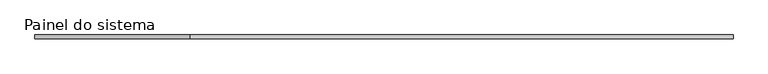
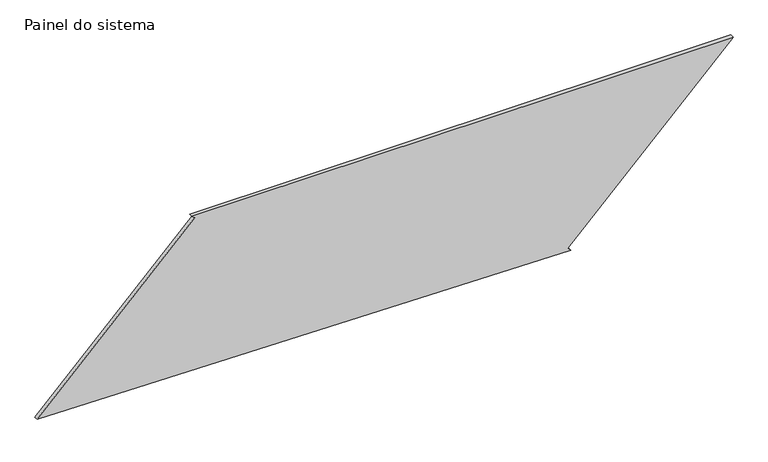
"""IFC4 building model written with IfcOpenShell, lengths in millimetres: plate geometry, Painel do sistema : Envidraçado."""

from ifc_helpers import new_model, si_unit, frame, origin, place, context, project, spatial, polyline, outline, extrude, source, transform, mapped, element, save


def painel_do_sistema_7fcae657(model_context):
    return source(origin(), model_context, "Body", "SweptSolid", [
        extrude(outline(polyline([(0.0, 1232.7009426), (17.655268, 1215.0008999), (1119.0901228, 2313.6495275), (1119.0901228, -1284.6877558), (1101.4348548, -1266.9877131), (52.1186543, -2313.6495275), (0.0, 1232.7009426)])), frame((0.0, 24.5, 0.0), z_axis=(0.0, 1.0, 0.0), x_axis=(0.0, 0.0, 1.0)), (0.0, 0.0, 1.0), 25.0),
    ])


if __name__ == "__main__":
    model = new_model("IFC4")
    model_context = context("Model", 3, world=origin())
    ifc_project = project(units=[si_unit("LENGTHUNIT", "METRE", prefix="MILLI")], contexts=[model_context])
    site = spatial("IfcSite", under=ifc_project)
    building = spatial("IfcBuilding", under=site)
    placement = place(None, origin())
    painel_do_sistema_shape = painel_do_sistema_7fcae657(model_context)
    element("IfcPlate", 1, ObjectType="Painel do sistema : Envidraçado", at=placement, inside=building, context=model_context, shape_type="MappedRepresentation", body=[
        mapped(painel_do_sistema_shape, transform((0.0, 0.0, 0.0), x_axis=(1.0, 0.0, 0.0), y_axis=(0.0, 1.0, 0.0), z_axis=(0.0, 0.0, 1.0))),
    ])
    save(model, "model.ifc")

# Revit data of these elements
# Type "Painel do sistema : Envidraçado"
#   Construction Type Id = "GSP4R"
#   Analytic Construction = "Vidraça única Pilkington 1/8 pol"
#   Visual Light Transmittance = 0.9
#   Solar Heat Gain Coefficient = 0.86
#   Heat Transfer Coefficient (U) = 6.7069 W/(m²·K)
# Element 1 (IfcPlate, "Painel do sistema : Envidraçado")
#   Materials on its faces: "Vidro"
# Materials
#   "Vidro": class "Vidro", colour RGB 0 128 192, transparency 0.9, Description = "Vidro de sílica", Cost = 0
